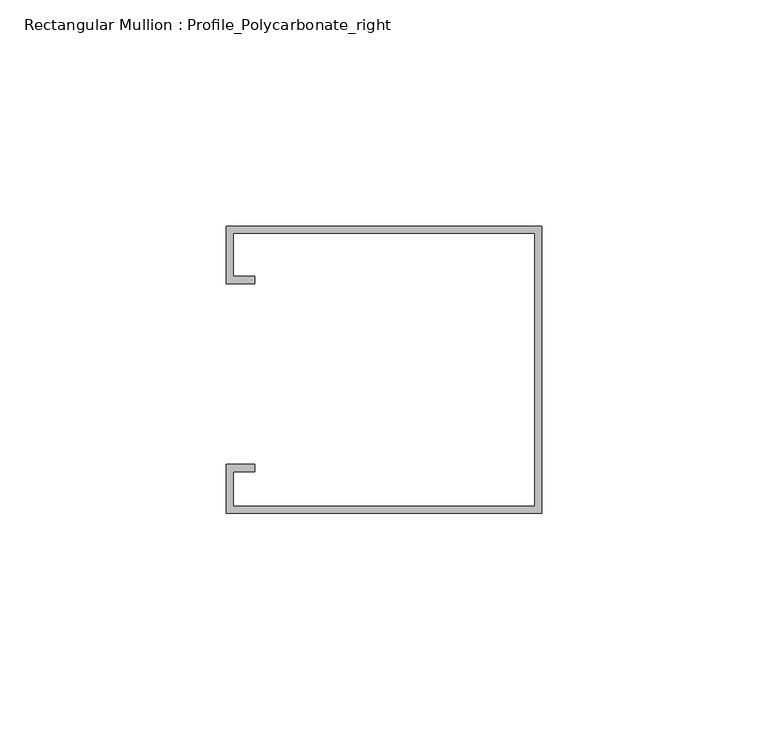
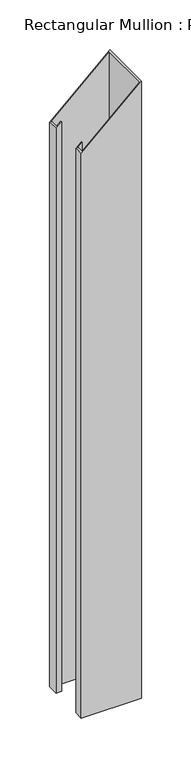
"""IFC4 building model written with IfcOpenShell, lengths in millimetres: member geometry, Rectangular Mullion : Profile_Polycarbonate_right."""

import ifcopenshell
import ifcopenshell.guid

model = None  # the IFC model being written
_history = None  # IfcOwnerHistory: only IFC2X3 demands one
_inside = {}  # id of a spatial element -> (the spatial element, [elements in it])
_under = {}  # id of a project, library or spatial element -> (it, [spatial elements below it])
_declared = {}  # id of a project -> (the project, [libraries it declares])
_typed = {}  # id of a type object -> (the type object, [elements of that type])
_made_of = {}  # id of a material, layer set ... -> (it, [elements and type objects made of it])


def new_model(schema):
    """Start an empty IFC model of exactly this schema.

    Asked for "IFC4X3", IfcOpenShell would pick the latest addendum, in which some entities
    have other attributes; the version numbers below select the first issue.
    IFC2X3 requires an IfcOwnerHistory on every rooted entity: one is made here for all.
    """
    global model, _history
    if schema == "IFC4X3":
        model = ifcopenshell.file(schema_version=(4, 3, 0, 0))
    else:
        model = ifcopenshell.file(schema=schema)
    _inside.clear()
    _under.clear()
    _declared.clear()
    _typed.clear()
    _made_of.clear()
    _history = None
    if model.schema == "IFC2X3":
        org = make("IfcOrganization", Name="unknown")
        user = make(
            "IfcPersonAndOrganization",
            ThePerson=make("IfcPerson", FamilyName="unknown"),
            TheOrganization=org,
        )
        app = make(
            "IfcApplication",
            ApplicationDeveloper=org,
            Version="unknown",
            ApplicationFullName="unknown",
            ApplicationIdentifier="unknown",
        )
        _history = make(
            "IfcOwnerHistory",
            OwningUser=user,
            OwningApplication=app,
            ChangeAction="ADDED",
            CreationDate=0,
        )
    return model


def make(cls, **values):
    """One entity of the class cls with the attributes given. An attribute that is None is left unset."""
    return model.create_entity(
        cls, **{name: value for name, value in values.items() if value is not None}
    )


def rooted(cls, **values):
    """An entity with a GlobalId (a new one), such as an element, a storey or a relation."""
    return make(cls, GlobalId=ifcopenshell.guid.new(), OwnerHistory=_history, **values)


def si_unit(unit_type, name, prefix=None):
    """IfcSIUnit, for example si_unit("LENGTHUNIT", "METRE", prefix="MILLI")."""
    return make("IfcSIUnit", UnitType=unit_type, Prefix=prefix, Name=name)


def assignment(units):
    """IfcUnitAssignment: the units of a project."""
    return None if units is None else make("IfcUnitAssignment", Units=units)


def point(xyz):
    """IfcCartesianPoint."""
    return None if xyz is None else make("IfcCartesianPoint", Coordinates=xyz)


def direction(xyz):
    """IfcDirection."""
    return None if xyz is None else make("IfcDirection", DirectionRatios=xyz)


def frame(location, z_axis=None, x_axis=None):
    """IfcAxis2Placement3D, a coordinate frame: its origin and axes. An axis left out is left unset."""
    return make(
        "IfcAxis2Placement3D",
        Location=point(location),
        Axis=direction(z_axis),
        RefDirection=direction(x_axis),
    )


def origin():
    """The frame at (0, 0, 0) with its axes left unset."""
    return frame((0.0, 0.0, 0.0))


def place(relative_to, where):
    """IfcLocalPlacement: puts the frame where relative to a parent placement (None: the world)."""
    return make(
        "IfcLocalPlacement", PlacementRelTo=relative_to, RelativePlacement=where
    )


def context(
    kind, dimensions, precision=None, world=None, true_north=None, identifier=None
):
    """IfcGeometricRepresentationContext, for example the 3D "Model" context."""
    return make(
        "IfcGeometricRepresentationContext",
        ContextIdentifier=identifier,
        ContextType=kind,
        CoordinateSpaceDimension=dimensions,
        Precision=precision,
        WorldCoordinateSystem=world,
        TrueNorth=true_north,
    )


def project(units=None, contexts=None):
    """IfcProject with its units and contexts."""
    return rooted(
        "IfcProject",
        Name="project",
        RepresentationContexts=contexts,
        UnitsInContext=assignment(units),
    )


def spatial(cls, under=None, at=None, **own):
    """A site, building, storey or space (cls), placed at a placement, below another one or the project."""
    s = rooted(cls, ObjectPlacement=at, **own)
    if under is not None:
        _under.setdefault(under.id(), (under, []))[1].append(s)
    return s


def faces_of(points, faces, orient=None, outer=None):
    """IfcFace entities. A face is a list of loops; a loop is a list of indices into points, from 0.

    orient and outer hold one flag for each loop. By default every Orientation is true, the
    first loop of a face is its IfcFaceOuterBound and the others are IfcFaceBound.
    """
    made = []
    for i, loops in enumerate(faces):
        bounds = []
        for j, loop in enumerate(loops):
            is_outer = j == 0 if outer is None else outer[i][j]
            bounds.append(
                make(
                    "IfcFaceOuterBound" if is_outer else "IfcFaceBound",
                    Bound=make("IfcPolyLoop", Polygon=[points[k] for k in loop]),
                    Orientation=True if orient is None else orient[i][j],
                )
            )
        made.append(make("IfcFace", Bounds=bounds))
    return made


def faceted_brep(points, faces, orient=None, outer=None, voids=None):
    """IfcFacetedBrep: a solid bounded by flat faces; with voids (closed shells), ...WithVoids."""
    shared = [point(p) for p in points]
    hull = make("IfcClosedShell", CfsFaces=faces_of(shared, faces, orient, outer))
    if voids is None:
        return make("IfcFacetedBrep", Outer=hull)
    return make(
        "IfcFacetedBrepWithVoids",
        Outer=hull,
        Voids=[
            make(cls, CfsFaces=faces_of(shared, fs, o, b)) for cls, fs, o, b in voids
        ],
    )


def shape(context_of_items, identifier, shape_type, items):
    """IfcShapeRepresentation: the items that make up one representation, for example the "Body"."""
    return make(
        "IfcShapeRepresentation",
        ContextOfItems=context_of_items,
        RepresentationIdentifier=identifier,
        RepresentationType=shape_type,
        Items=items,
    )


def source(mapping_origin, context_of_items, identifier, shape_type, items):
    """IfcRepresentationMap: a shape defined once, which mapped items show again and again."""
    return make(
        "IfcRepresentationMap",
        MappingOrigin=mapping_origin,
        MappedRepresentation=shape(context_of_items, identifier, shape_type, items),
    )


def transform(
    local_origin,
    x_axis=None,
    y_axis=None,
    z_axis=None,
    scale=None,
    scale2=None,
    scale3=None,
    uniform=True,
):
    """IfcCartesianTransformationOperator3D, or its non-uniform kind. x_axis, y_axis, z_axis: its Axis1, 2, 3."""
    if uniform:
        return make(
            "IfcCartesianTransformationOperator3D",
            Axis1=direction(x_axis),
            Axis2=direction(y_axis),
            LocalOrigin=point(local_origin),
            Scale=scale,
            Axis3=direction(z_axis),
        )
    return make(
        "IfcCartesianTransformationOperator3DnonUniform",
        Axis1=direction(x_axis),
        Axis2=direction(y_axis),
        LocalOrigin=point(local_origin),
        Scale=scale,
        Axis3=direction(z_axis),
        Scale2=scale2,
        Scale3=scale3,
    )


def mapped(mapping_source, mapping_target):
    """IfcMappedItem: shows the shape of a source again, moved by a transform."""
    return make(
        "IfcMappedItem", MappingSource=mapping_source, MappingTarget=mapping_target
    )


def made_of(thing, what):
    """Note that an element or type object is made of a material, layer set ...; save() writes the relation."""
    if what is not None:
        _made_of.setdefault(what.id(), (what, []))[1].append(thing)
    return thing


def element(
    cls,
    number,
    at=None,
    inside=None,
    cuts=None,
    type_object=None,
    material=None,
    context=None,
    identifier="Body",
    shape_type=None,
    held_by="IfcProductDefinitionShape",
    body=None,
    shapes=None,
    **own,
):
    """One element of the class cls, such as IfcWall. Its Tag is "e" and its number.

    at: its placement. inside: the storey or other place that contains it. cuts: it is an
    opening in that element (IfcRelVoidsElement). A single representation is given by context,
    identifier, shape_type and body (its items); several are given by shapes. held_by: the class
    of the entity that holds the representations. save() writes the other relations.
    """
    e = rooted(cls, Tag="e%d" % number, ObjectPlacement=at, **own)
    if body is not None:
        shapes = [shape(context, identifier, shape_type, body)]
    if shapes is not None:
        e.Representation = make(held_by, Representations=shapes)
    if inside is not None:
        _inside.setdefault(inside.id(), (inside, []))[1].append(e)
    if cuts is not None:
        rooted(
            "IfcRelVoidsElement", RelatingBuildingElement=cuts, RelatedOpeningElement=e
        )
    if type_object is not None:
        _typed.setdefault(type_object.id(), (type_object, []))[1].append(e)
    return made_of(e, material)


def aggregate(whole, parts):
    """IfcRelAggregates: a whole, such as a stair, and the parts it consists of."""
    return rooted("IfcRelAggregates", RelatingObject=whole, RelatedObjects=parts)


def save(model, path):
    """Write the relations noted so far, then the file.

    IfcRelAggregates (storeys below a building ...), IfcRelContainedInSpatialStructure (elements
    in a storey), IfcRelDefinesByType, IfcRelAssociatesMaterial and IfcRelDeclares: one each for
    every whole, place, type object, material and project.
    """
    for whole, parts in _under.values():
        aggregate(whole, parts)
    for where, things in _inside.values():
        rooted(
            "IfcRelContainedInSpatialStructure",
            RelatedElements=things,
            RelatingStructure=where,
        )
    for kind, things in _typed.values():
        rooted("IfcRelDefinesByType", RelatedObjects=things, RelatingType=kind)
    for what, things in _made_of.values():
        rooted("IfcRelAssociatesMaterial", RelatedObjects=things, RelatingMaterial=what)
    for by, libraries in _declared.values():
        rooted("IfcRelDeclares", RelatingContext=by, RelatedDefinitions=libraries)
    model.write(path)


def rectangular_mullion_profile_polycarbonate_right_fcc73ad3(model_context):
    return source(origin(), model_context, "Body", "Brep", [
        faceted_brep([(0.0, 32.7, -756.1791667), (0.0, -30.8, -756.1791667), (-69.85, -30.8, -756.1791667), (-69.85, -20.0, -756.1791667), (-63.5, -20.0, -756.1791667), (-63.5, -21.5875, -756.1791667), (-68.2625, -21.5875, -756.1791667), (-68.2625, -29.2125, -756.1791667), (-1.5875, -29.2125, -756.1791667), (-1.5875, 31.1125, -756.1791667), (-68.2625, 31.1125, -756.1791667), (-68.2625, 21.5875, -756.1791667), (-63.5, 21.5875, -756.1791667), (-63.5, 20.0, -756.1791667), (-69.85, 20.0, -756.1791667), (-69.85, 32.7, -756.1791667), (-69.85, 32.7, -64.2712818), (0.0, 32.7, 0.0), (-69.85, 20.0, -64.2712818), (-63.5, 20.0, -58.428438), (-63.5, 21.5875, -58.428438), (-68.2625, 21.5875, -62.8105708), (-68.2625, 31.1125, -62.8105708), (-1.5875, 31.1125, -1.4607109), (-1.5875, -29.2125, -1.4607109), (-68.2625, -29.2125, -62.8105708), (-68.2625, -21.5875, -62.8105708), (-63.5, -21.5875, -58.428438), (-63.5, -20.0, -58.428438), (-69.85, -20.0, -64.2712818), (-69.85, -30.8, -64.2712818), (0.0, -30.8, 0.0)], [[[0, 1, 2, 3, 4, 5, 6, 7, 8, 9, 10, 11, 12, 13, 14, 15]], [[16, 17, 0, 15]], [[18, 16, 15, 14]], [[19, 18, 14, 13]], [[20, 19, 13, 12]], [[21, 20, 12, 11]], [[22, 21, 11, 10]], [[23, 22, 10, 9]], [[24, 23, 9, 8]], [[25, 24, 8, 7]], [[26, 25, 7, 6]], [[27, 26, 6, 5]], [[28, 27, 5, 4]], [[29, 28, 4, 3]], [[30, 29, 3, 2]], [[31, 30, 2, 1]], [[17, 31, 1, 0]], [[17, 16, 18, 19, 20, 21, 22, 23, 24, 25, 26, 27, 28, 29, 30, 31]]]),
    ])


if __name__ == "__main__":
    model = new_model("IFC4")
    model_context = context("Model", 3, world=origin())
    ifc_project = project(units=[si_unit("LENGTHUNIT", "METRE", prefix="MILLI")], contexts=[model_context])
    site = spatial("IfcSite", under=ifc_project)
    building = spatial("IfcBuilding", under=site)
    placement = place(None, origin())
    rectangular_mullion_profile_polycarbonate_right_shape = rectangular_mullion_profile_polycarbonate_right_fcc73ad3(model_context)
    element("IfcMember", 1, ObjectType="Rectangular Mullion : Profile_Polycarbonate_right", at=placement, inside=building, context=model_context, shape_type="MappedRepresentation", body=[
        mapped(rectangular_mullion_profile_polycarbonate_right_shape, transform((0.0, 0.0, 0.0), x_axis=(1.0, 0.0, 0.0), y_axis=(0.0, 1.0, 0.0), z_axis=(0.0, 0.0, 1.0))),
    ])
    save(model, "model.ifc")

# Revit data of these elements
# Type "Rectangular Mullion : Profile_Polycarbonate_right"
#   built-in parameter 1007322 = 0.208333 (stored number, unit not read)
#   built-in parameter 1007321 = 0 (stored number, unit not read)
#   built-in parameter 1007320 = 0.00520833 (stored number, unit not read)
# Element 1 (IfcMember, "Rectangular Mullion : Profile_Polycarbonate_right")
#   Materials on its faces: "ALUMINUM PROFILE AT POLYCARBONATE PANEL"
# Materials
#   "ALUMINUM PROFILE AT POLYCARBONATE PANEL": class "Metal", colour RGB 244 244 244, transparency 0, Description = "Aluminum 6061", Cost = 0
